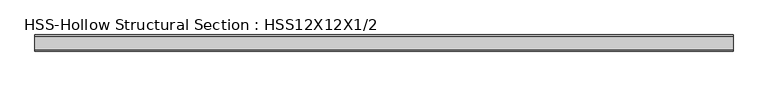
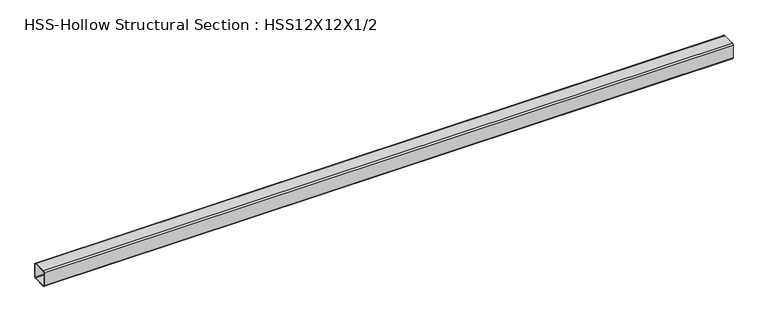
"""IFC4 building model written with IfcOpenShell, lengths in millimetres: beam geometry, HSS-Hollow Structural Section : HSS12X12X1/2."""

from ifc_helpers import new_model, si_unit, point, frame, frame_2d, origin, place, context, project, spatial, polyline, circle_curve, trimmed, segment, composite_curve, outline, extrude, source, transform, mapped, element, save


def hss_hollow_structural_section_hss12x12x1_2_ac1cf4bf(model_context):
    return source(origin(), model_context, "Body", "SweptSolid", [
        extrude(outline(composite_curve([segment(polyline([(152.4, 128.778), (152.4, -128.778)]), True, "CONTINUOUS"), segment(trimmed(circle_curve(frame_2d((128.778, -128.778)), 23.622), [point((152.4, -128.778))], [point((128.778, -152.4))], False, "CARTESIAN"), True, "CONTINUOUS"), segment(polyline([(128.778, -152.4), (-128.778, -152.4)]), True, "CONTINUOUS"), segment(trimmed(circle_curve(frame_2d((-128.778, -128.778)), 23.622), [point((-128.778, -152.4))], [point((-152.4, -128.778))], False, "CARTESIAN"), True, "CONTINUOUS"), segment(polyline([(-152.4, -128.778), (-152.4, 128.778)]), True, "CONTINUOUS"), segment(trimmed(circle_curve(frame_2d((-128.778, 128.778)), 23.622), [point((-152.4, 128.778))], [point((-128.778, 152.4))], False, "CARTESIAN"), True, "CONTINUOUS"), segment(polyline([(-128.778, 152.4), (128.778, 152.4)]), True, "CONTINUOUS"), segment(trimmed(circle_curve(frame_2d((128.778, 128.778)), 23.622), [point((128.778, 152.4))], [point((152.4, 128.778))], False, "CARTESIAN"), True, "CONTINUOUS")], self_intersect=False), holes=[composite_curve([segment(trimmed(circle_curve(frame_2d((-128.778, 128.778)), 11.811), [point((-128.778, 140.589))], [point((-140.589, 128.778))], True, "CARTESIAN"), True, "CONTINUOUS"), segment(polyline([(-140.589, 128.778), (-140.589, -128.778)]), True, "CONTINUOUS"), segment(trimmed(circle_curve(frame_2d((-128.778, -128.778)), 11.811), [point((-140.589, -128.778))], [point((-128.778, -140.589))], True, "CARTESIAN"), True, "CONTINUOUS"), segment(polyline([(-128.778, -140.589), (128.778, -140.589)]), True, "CONTINUOUS"), segment(trimmed(circle_curve(frame_2d((128.778, -128.778)), 11.811), [point((128.778, -140.589))], [point((140.589, -128.778))], True, "CARTESIAN"), True, "CONTINUOUS"), segment(polyline([(140.589, -128.778), (140.589, 128.778)]), True, "CONTINUOUS"), segment(trimmed(circle_curve(frame_2d((128.778, 128.778)), 11.811), [point((140.589, 128.778))], [point((128.778, 140.589))], True, "CARTESIAN"), True, "CONTINUOUS"), segment(polyline([(128.778, 140.589), (-128.778, 140.589)]), True, "CONTINUOUS")], self_intersect=False)]), frame((-6674.2846052, 0.0, 0.0), z_axis=(1.0, 0.0, 0.0), x_axis=(0.0, 1.0, 0.0)), (0.0, 0.0, 1.0), 13185.2516923),
    ])


if __name__ == "__main__":
    model = new_model("IFC4")
    model_context = context("Model", 3, world=origin())
    ifc_project = project(units=[si_unit("LENGTHUNIT", "METRE", prefix="MILLI")], contexts=[model_context])
    site = spatial("IfcSite", under=ifc_project)
    building = spatial("IfcBuilding", under=site)
    placement = place(None, origin())
    hss_hollow_structural_section_hss12x12x1_2_shape = hss_hollow_structural_section_hss12x12x1_2_ac1cf4bf(model_context)
    element("IfcBeam", 1, ObjectType="HSS-Hollow Structural Section : HSS12X12X1/2", at=placement, inside=building, context=model_context, shape_type="MappedRepresentation", body=[
        mapped(hss_hollow_structural_section_hss12x12x1_2_shape, transform((0.0, 0.0, 0.0), x_axis=(1.0, 0.0, 0.0), y_axis=(0.0, 1.0, 0.0), z_axis=(0.0, 0.0, 1.0))),
    ])
    save(model, "model.ifc")

# Revit data of these elements
# Type "HSS-Hollow Structural Section : HSS12X12X1/2"
#   Assembly Code = "B10"
#   Shape = "Square"
#   W = 75.9
#   Ht = 304.8 mm
#   Length [instance default] = 1524 mm
#   b = 304.8 mm
#   kr = 23.622 mm
#   t = 11.811 mm
#   A = 0.0134838 m²
#   Structural Material [instance default] = Steel ASTM A500, Grade B, Rectangular and Square
# Element 1 (IfcBeam, "HSS-Hollow Structural Section : HSS12X12X1/2")
#   Structural Material = Aluminum 7175 T73 0 Hot Formed
#   Materials on its faces: "Aluminum 7175 T73 0 Hot Formed"
# Materials
#   "Steel ASTM A500, Grade B, Rectangular and Square": class "Metal", colour RGB 199 199 199, transparency 0, Description = "Carbon steel", Cost = 0
#   "Aluminum 7175 T73 0 Hot Formed": class "Metal", colour RGB 120 120 120, transparency 0, Description = "Physical material.", Cost = 0
